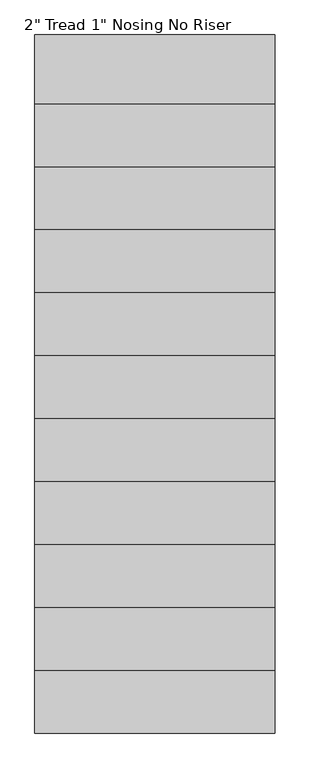
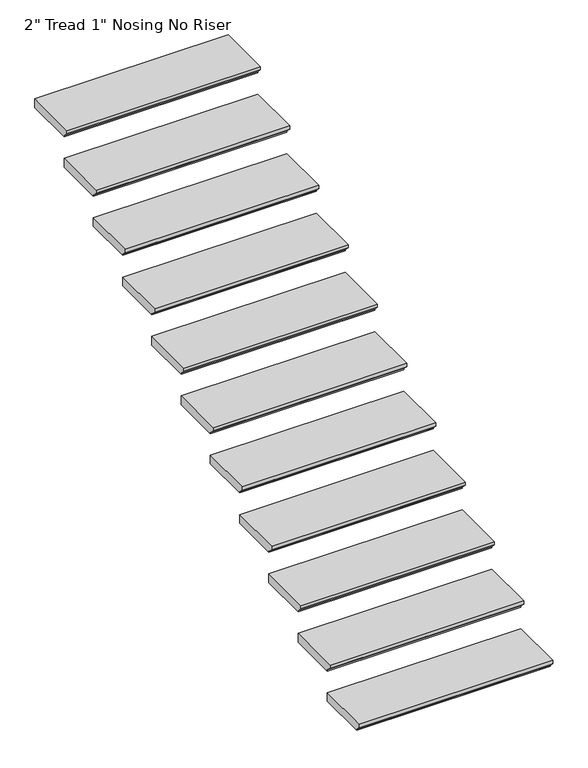
"""IFC4 building model written with IfcOpenShell, lengths in millimetres: stair flight geometry."""

import ifcopenshell
import ifcopenshell.guid

model = None  # the IFC model being written
_history = None  # IfcOwnerHistory: only IFC2X3 demands one
_inside = {}  # id of a spatial element -> (the spatial element, [elements in it])
_under = {}  # id of a project, library or spatial element -> (it, [spatial elements below it])
_declared = {}  # id of a project -> (the project, [libraries it declares])
_typed = {}  # id of a type object -> (the type object, [elements of that type])
_made_of = {}  # id of a material, layer set ... -> (it, [elements and type objects made of it])


def new_model(schema):
    """Start an empty IFC model of exactly this schema.

    Asked for "IFC4X3", IfcOpenShell would pick the latest addendum, in which some entities
    have other attributes; the version numbers below select the first issue.
    IFC2X3 requires an IfcOwnerHistory on every rooted entity: one is made here for all.
    """
    global model, _history
    if schema == "IFC4X3":
        model = ifcopenshell.file(schema_version=(4, 3, 0, 0))
    else:
        model = ifcopenshell.file(schema=schema)
    _inside.clear()
    _under.clear()
    _declared.clear()
    _typed.clear()
    _made_of.clear()
    _history = None
    if model.schema == "IFC2X3":
        org = make("IfcOrganization", Name="unknown")
        user = make(
            "IfcPersonAndOrganization",
            ThePerson=make("IfcPerson", FamilyName="unknown"),
            TheOrganization=org,
        )
        app = make(
            "IfcApplication",
            ApplicationDeveloper=org,
            Version="unknown",
            ApplicationFullName="unknown",
            ApplicationIdentifier="unknown",
        )
        _history = make(
            "IfcOwnerHistory",
            OwningUser=user,
            OwningApplication=app,
            ChangeAction="ADDED",
            CreationDate=0,
        )
    return model


def make(cls, **values):
    """One entity of the class cls with the attributes given. An attribute that is None is left unset."""
    return model.create_entity(
        cls, **{name: value for name, value in values.items() if value is not None}
    )


def rooted(cls, **values):
    """An entity with a GlobalId (a new one), such as an element, a storey or a relation."""
    return make(cls, GlobalId=ifcopenshell.guid.new(), OwnerHistory=_history, **values)


def si_unit(unit_type, name, prefix=None):
    """IfcSIUnit, for example si_unit("LENGTHUNIT", "METRE", prefix="MILLI")."""
    return make("IfcSIUnit", UnitType=unit_type, Prefix=prefix, Name=name)


def assignment(units):
    """IfcUnitAssignment: the units of a project."""
    return None if units is None else make("IfcUnitAssignment", Units=units)


def point(xyz):
    """IfcCartesianPoint."""
    return None if xyz is None else make("IfcCartesianPoint", Coordinates=xyz)


def direction(xyz):
    """IfcDirection."""
    return None if xyz is None else make("IfcDirection", DirectionRatios=xyz)


def frame(location, z_axis=None, x_axis=None):
    """IfcAxis2Placement3D, a coordinate frame: its origin and axes. An axis left out is left unset."""
    return make(
        "IfcAxis2Placement3D",
        Location=point(location),
        Axis=direction(z_axis),
        RefDirection=direction(x_axis),
    )


def origin():
    """The frame at (0, 0, 0) with its axes left unset."""
    return frame((0.0, 0.0, 0.0))


def place(relative_to, where):
    """IfcLocalPlacement: puts the frame where relative to a parent placement (None: the world)."""
    return make(
        "IfcLocalPlacement", PlacementRelTo=relative_to, RelativePlacement=where
    )


def context(
    kind, dimensions, precision=None, world=None, true_north=None, identifier=None
):
    """IfcGeometricRepresentationContext, for example the 3D "Model" context."""
    return make(
        "IfcGeometricRepresentationContext",
        ContextIdentifier=identifier,
        ContextType=kind,
        CoordinateSpaceDimension=dimensions,
        Precision=precision,
        WorldCoordinateSystem=world,
        TrueNorth=true_north,
    )


def project(units=None, contexts=None):
    """IfcProject with its units and contexts."""
    return rooted(
        "IfcProject",
        Name="project",
        RepresentationContexts=contexts,
        UnitsInContext=assignment(units),
    )


def spatial(cls, under=None, at=None, **own):
    """A site, building, storey or space (cls), placed at a placement, below another one or the project."""
    s = rooted(cls, ObjectPlacement=at, **own)
    if under is not None:
        _under.setdefault(under.id(), (under, []))[1].append(s)
    return s


def faces_of(points, faces, orient=None, outer=None):
    """IfcFace entities. A face is a list of loops; a loop is a list of indices into points, from 0.

    orient and outer hold one flag for each loop. By default every Orientation is true, the
    first loop of a face is its IfcFaceOuterBound and the others are IfcFaceBound.
    """
    made = []
    for i, loops in enumerate(faces):
        bounds = []
        for j, loop in enumerate(loops):
            is_outer = j == 0 if outer is None else outer[i][j]
            bounds.append(
                make(
                    "IfcFaceOuterBound" if is_outer else "IfcFaceBound",
                    Bound=make("IfcPolyLoop", Polygon=[points[k] for k in loop]),
                    Orientation=True if orient is None else orient[i][j],
                )
            )
        made.append(make("IfcFace", Bounds=bounds))
    return made


def faceted_brep(points, faces, orient=None, outer=None, voids=None):
    """IfcFacetedBrep: a solid bounded by flat faces; with voids (closed shells), ...WithVoids."""
    shared = [point(p) for p in points]
    hull = make("IfcClosedShell", CfsFaces=faces_of(shared, faces, orient, outer))
    if voids is None:
        return make("IfcFacetedBrep", Outer=hull)
    return make(
        "IfcFacetedBrepWithVoids",
        Outer=hull,
        Voids=[
            make(cls, CfsFaces=faces_of(shared, fs, o, b)) for cls, fs, o, b in voids
        ],
    )


def shape(context_of_items, identifier, shape_type, items):
    """IfcShapeRepresentation: the items that make up one representation, for example the "Body"."""
    return make(
        "IfcShapeRepresentation",
        ContextOfItems=context_of_items,
        RepresentationIdentifier=identifier,
        RepresentationType=shape_type,
        Items=items,
    )


def source(mapping_origin, context_of_items, identifier, shape_type, items):
    """IfcRepresentationMap: a shape defined once, which mapped items show again and again."""
    return make(
        "IfcRepresentationMap",
        MappingOrigin=mapping_origin,
        MappedRepresentation=shape(context_of_items, identifier, shape_type, items),
    )


def transform(
    local_origin,
    x_axis=None,
    y_axis=None,
    z_axis=None,
    scale=None,
    scale2=None,
    scale3=None,
    uniform=True,
):
    """IfcCartesianTransformationOperator3D, or its non-uniform kind. x_axis, y_axis, z_axis: its Axis1, 2, 3."""
    if uniform:
        return make(
            "IfcCartesianTransformationOperator3D",
            Axis1=direction(x_axis),
            Axis2=direction(y_axis),
            LocalOrigin=point(local_origin),
            Scale=scale,
            Axis3=direction(z_axis),
        )
    return make(
        "IfcCartesianTransformationOperator3DnonUniform",
        Axis1=direction(x_axis),
        Axis2=direction(y_axis),
        LocalOrigin=point(local_origin),
        Scale=scale,
        Axis3=direction(z_axis),
        Scale2=scale2,
        Scale3=scale3,
    )


def mapped(mapping_source, mapping_target):
    """IfcMappedItem: shows the shape of a source again, moved by a transform."""
    return make(
        "IfcMappedItem", MappingSource=mapping_source, MappingTarget=mapping_target
    )


def made_of(thing, what):
    """Note that an element or type object is made of a material, layer set ...; save() writes the relation."""
    if what is not None:
        _made_of.setdefault(what.id(), (what, []))[1].append(thing)
    return thing


def element(
    cls,
    number,
    at=None,
    inside=None,
    cuts=None,
    type_object=None,
    material=None,
    context=None,
    identifier="Body",
    shape_type=None,
    held_by="IfcProductDefinitionShape",
    body=None,
    shapes=None,
    **own,
):
    """One element of the class cls, such as IfcWall. Its Tag is "e" and its number.

    at: its placement. inside: the storey or other place that contains it. cuts: it is an
    opening in that element (IfcRelVoidsElement). A single representation is given by context,
    identifier, shape_type and body (its items); several are given by shapes. held_by: the class
    of the entity that holds the representations. save() writes the other relations.
    """
    e = rooted(cls, Tag="e%d" % number, ObjectPlacement=at, **own)
    if body is not None:
        shapes = [shape(context, identifier, shape_type, body)]
    if shapes is not None:
        e.Representation = make(held_by, Representations=shapes)
    if inside is not None:
        _inside.setdefault(inside.id(), (inside, []))[1].append(e)
    if cuts is not None:
        rooted(
            "IfcRelVoidsElement", RelatingBuildingElement=cuts, RelatedOpeningElement=e
        )
    if type_object is not None:
        _typed.setdefault(type_object.id(), (type_object, []))[1].append(e)
    return made_of(e, material)


def aggregate(whole, parts):
    """IfcRelAggregates: a whole, such as a stair, and the parts it consists of."""
    return rooted("IfcRelAggregates", RelatingObject=whole, RelatedObjects=parts)


def save(model, path):
    """Write the relations noted so far, then the file.

    IfcRelAggregates (storeys below a building ...), IfcRelContainedInSpatialStructure (elements
    in a storey), IfcRelDefinesByType, IfcRelAssociatesMaterial and IfcRelDeclares: one each for
    every whole, place, type object, material and project.
    """
    for whole, parts in _under.values():
        aggregate(whole, parts)
    for where, things in _inside.values():
        rooted(
            "IfcRelContainedInSpatialStructure",
            RelatedElements=things,
            RelatingStructure=where,
        )
    for kind, things in _typed.values():
        rooted("IfcRelDefinesByType", RelatedObjects=things, RelatingType=kind)
    for what, things in _made_of.values():
        rooted("IfcRelAssociatesMaterial", RelatedObjects=things, RelatingMaterial=what)
    for by, libraries in _declared.values():
        rooted("IfcRelDeclares", RelatingContext=by, RelatedDefinitions=libraries)
    model.write(path)


def stair_flight_8578e766(model_context):
    return source(origin(), model_context, "Body", "Brep", [
        faceted_brep([(-7676.1954607, -1875.4304995, 30637.6456522), (-7676.1954607, -1875.4304995, 30656.6956522), (-8742.9954607, -1875.4304995, 30656.6956522), (-8742.9954607, -1875.4304995, 30637.6456522), (-7676.1954607, -1850.0304995, 30612.2456522), (-8742.9954607, -1850.0304995, 30612.2456522), (-7676.1954607, -1570.6304995, 30656.6956522), (-8742.9954607, -1570.6304995, 30656.6956522), (-8742.9954607, -1850.0304995, 30605.8956522), (-8742.9954607, -1570.6304995, 30605.8956522), (-7676.1954607, -1570.6304995, 30605.8956522), (-7676.1954607, -1850.0304995, 30605.8956522)], [[[0, 1, 2, 3]], [[4, 0, 3, 5]], [[2, 1, 6, 7]], [[8, 9, 10, 11]], [[2, 7, 9, 8, 5, 3]], [[8, 11, 4, 5]], [[6, 1, 0, 4, 11, 10]], [[7, 6, 10, 9]]]),
        faceted_brep([(-8742.9954607, -1596.0304995, 30833.3913043), (-7676.1954607, -1596.0304995, 30833.3913043), (-7676.1954607, -1291.2304995, 30833.3913043), (-8742.9954607, -1291.2304995, 30833.3913043), (-8742.9954607, -1570.6304995, 30782.5913043), (-8742.9954607, -1291.2304995, 30782.5913043), (-7676.1954607, -1291.2304995, 30782.5913043), (-7676.1954607, -1570.6304995, 30782.5913043), (-8742.9954607, -1570.6304995, 30788.9413043), (-8742.9954607, -1596.0304995, 30814.3413043), (-7676.1954607, -1570.6304995, 30788.9413043), (-7676.1954607, -1596.0304995, 30814.3413043)], [[[0, 1, 2, 3]], [[4, 5, 6, 7]], [[0, 3, 5, 4, 8, 9]], [[4, 7, 10, 8]], [[2, 1, 11, 10, 7, 6]], [[3, 2, 6, 5]], [[11, 1, 0, 9]], [[10, 11, 9, 8]]]),
        faceted_brep([(-8742.9954607, -1316.6304995, 31010.0869565), (-7676.1954607, -1316.6304995, 31010.0869565), (-7676.1954607, -1011.8304995, 31010.0869565), (-8742.9954607, -1011.8304995, 31010.0869565), (-8742.9954607, -1291.2304995, 30959.2869565), (-8742.9954607, -1011.8304995, 30959.2869565), (-7676.1954607, -1011.8304995, 30959.2869565), (-7676.1954607, -1291.2304995, 30959.2869565), (-8742.9954607, -1291.2304995, 30965.6369565), (-8742.9954607, -1316.6304995, 30991.0369565), (-7676.1954607, -1291.2304995, 30965.6369565), (-7676.1954607, -1316.6304995, 30991.0369565)], [[[0, 1, 2, 3]], [[4, 5, 6, 7]], [[0, 3, 5, 4, 8, 9]], [[4, 7, 10, 8]], [[2, 1, 11, 10, 7, 6]], [[3, 2, 6, 5]], [[11, 1, 0, 9]], [[10, 11, 9, 8]]]),
        faceted_brep([(-8742.9954607, -1037.2304995, 31186.7826087), (-7676.1954607, -1037.2304995, 31186.7826087), (-7676.1954607, -732.4304995, 31186.7826087), (-8742.9954607, -732.4304995, 31186.7826087), (-8742.9954607, -1011.8304995, 31135.9826087), (-8742.9954607, -732.4304995, 31135.9826087), (-7676.1954607, -732.4304995, 31135.9826087), (-7676.1954607, -1011.8304995, 31135.9826087), (-8742.9954607, -1011.8304995, 31142.3326087), (-8742.9954607, -1037.2304995, 31167.7326087), (-7676.1954607, -1011.8304995, 31142.3326087), (-7676.1954607, -1037.2304995, 31167.7326087)], [[[0, 1, 2, 3]], [[4, 5, 6, 7]], [[0, 3, 5, 4, 8, 9]], [[4, 7, 10, 8]], [[2, 1, 11, 10, 7, 6]], [[3, 2, 6, 5]], [[11, 1, 0, 9]], [[10, 11, 9, 8]]]),
        faceted_brep([(-8742.9954607, -757.8304995, 31363.4782609), (-7676.1954607, -757.8304995, 31363.4782609), (-7676.1954607, -453.0304995, 31363.4782609), (-8742.9954607, -453.0304995, 31363.4782609), (-8742.9954607, -732.4304995, 31312.6782609), (-8742.9954607, -453.0304995, 31312.6782609), (-7676.1954607, -453.0304995, 31312.6782609), (-7676.1954607, -732.4304995, 31312.6782609), (-8742.9954607, -732.4304995, 31319.0282609), (-8742.9954607, -757.8304995, 31344.4282609), (-7676.1954607, -732.4304995, 31319.0282609), (-7676.1954607, -757.8304995, 31344.4282609)], [[[0, 1, 2, 3]], [[4, 5, 6, 7]], [[0, 3, 5, 4, 8, 9]], [[4, 7, 10, 8]], [[2, 1, 11, 10, 7, 6]], [[3, 2, 6, 5]], [[11, 1, 0, 9]], [[10, 11, 9, 8]]]),
        faceted_brep([(-8742.9954607, -478.4304995, 31540.173913), (-7676.1954607, -478.4304995, 31540.173913), (-7676.1954607, -173.6304995, 31540.173913), (-8742.9954607, -173.6304995, 31540.173913), (-8742.9954607, -453.0304995, 31489.373913), (-8742.9954607, -173.6304995, 31489.373913), (-7676.1954607, -173.6304995, 31489.373913), (-7676.1954607, -453.0304995, 31489.373913), (-8742.9954607, -453.0304995, 31495.723913), (-8742.9954607, -478.4304995, 31521.123913), (-7676.1954607, -453.0304995, 31495.723913), (-7676.1954607, -478.4304995, 31521.123913)], [[[0, 1, 2, 3]], [[4, 5, 6, 7]], [[0, 3, 5, 4, 8, 9]], [[4, 7, 10, 8]], [[2, 1, 11, 10, 7, 6]], [[3, 2, 6, 5]], [[11, 1, 0, 9]], [[10, 11, 9, 8]]]),
        faceted_brep([(-8742.9954607, -199.0304995, 31716.8695652), (-7676.1954607, -199.0304995, 31716.8695652), (-7676.1954607, 105.7695005, 31716.8695652), (-8742.9954607, 105.7695005, 31716.8695652), (-8742.9954607, -173.6304995, 31666.0695652), (-8742.9954607, 105.7695005, 31666.0695652), (-7676.1954607, 105.7695005, 31666.0695652), (-7676.1954607, -173.6304995, 31666.0695652), (-8742.9954607, -173.6304995, 31672.4195652), (-8742.9954607, -199.0304995, 31697.8195652), (-7676.1954607, -173.6304995, 31672.4195652), (-7676.1954607, -199.0304995, 31697.8195652)], [[[0, 1, 2, 3]], [[4, 5, 6, 7]], [[0, 3, 5, 4, 8, 9]], [[4, 7, 10, 8]], [[2, 1, 11, 10, 7, 6]], [[3, 2, 6, 5]], [[11, 1, 0, 9]], [[10, 11, 9, 8]]]),
        faceted_brep([(-8742.9954607, 80.3695005, 31893.5652174), (-7676.1954607, 80.3695005, 31893.5652174), (-7676.1954607, 385.1695005, 31893.5652174), (-8742.9954607, 385.1695005, 31893.5652174), (-8742.9954607, 105.7695005, 31842.7652174), (-8742.9954607, 385.1695005, 31842.7652174), (-7676.1954607, 385.1695005, 31842.7652174), (-7676.1954607, 105.7695005, 31842.7652174), (-8742.9954607, 105.7695005, 31849.1152174), (-8742.9954607, 80.3695005, 31874.5152174), (-7676.1954607, 105.7695005, 31849.1152174), (-7676.1954607, 80.3695005, 31874.5152174)], [[[0, 1, 2, 3]], [[4, 5, 6, 7]], [[0, 3, 5, 4, 8, 9]], [[4, 7, 10, 8]], [[2, 1, 11, 10, 7, 6]], [[3, 2, 6, 5]], [[11, 1, 0, 9]], [[10, 11, 9, 8]]]),
        faceted_brep([(-8742.9954607, 359.7695005, 32070.2608696), (-7676.1954607, 359.7695005, 32070.2608696), (-7676.1954607, 664.5695005, 32070.2608696), (-8742.9954607, 664.5695005, 32070.2608696), (-8742.9954607, 385.1695005, 32019.4608696), (-8742.9954607, 664.5695005, 32019.4608696), (-7676.1954607, 664.5695005, 32019.4608696), (-7676.1954607, 385.1695005, 32019.4608696), (-8742.9954607, 385.1695005, 32025.8108696), (-8742.9954607, 359.7695005, 32051.2108696), (-7676.1954607, 385.1695005, 32025.8108696), (-7676.1954607, 359.7695005, 32051.2108696)], [[[0, 1, 2, 3]], [[4, 5, 6, 7]], [[0, 3, 5, 4, 8, 9]], [[4, 7, 10, 8]], [[2, 1, 11, 10, 7, 6]], [[3, 2, 6, 5]], [[11, 1, 0, 9]], [[10, 11, 9, 8]]]),
        faceted_brep([(-8742.9954607, 639.1695005, 32246.9565217), (-7676.1954607, 639.1695005, 32246.9565217), (-7676.1954607, 943.9695005, 32246.9565217), (-8742.9954607, 943.9695005, 32246.9565217), (-8742.9954607, 664.5695005, 32196.1565217), (-8742.9954607, 943.9695005, 32196.1565217), (-7676.1954607, 943.9695005, 32196.1565217), (-7676.1954607, 664.5695005, 32196.1565217), (-8742.9954607, 664.5695005, 32202.5065217), (-8742.9954607, 639.1695005, 32227.9065217), (-7676.1954607, 664.5695005, 32202.5065217), (-7676.1954607, 639.1695005, 32227.9065217)], [[[0, 1, 2, 3]], [[4, 5, 6, 7]], [[0, 3, 5, 4, 8, 9]], [[4, 7, 10, 8]], [[2, 1, 11, 10, 7, 6]], [[3, 2, 6, 5]], [[11, 1, 0, 9]], [[10, 11, 9, 8]]]),
        faceted_brep([(-8742.9954607, 918.5695005, 32423.6521739), (-7676.1954607, 918.5695005, 32423.6521739), (-7676.1954607, 1197.9695005, 32423.6521739), (-7676.1954607, 1223.3695005, 32423.6521739), (-8742.9954607, 1223.3695005, 32423.6521739), (-8742.9954607, 943.9695005, 32372.8521739), (-8742.9954607, 1223.3695005, 32372.8521739), (-7676.1954607, 1223.3695005, 32372.8521739), (-7676.1954607, 1197.9695005, 32372.8521739), (-7676.1954607, 943.9695005, 32372.8521739), (-8742.9954607, 943.9695005, 32379.2021739), (-8742.9954607, 918.5695005, 32404.6021739), (-7676.1954607, 943.9695005, 32379.2021739), (-7676.1954607, 918.5695005, 32404.6021739)], [[[0, 1, 2, 3, 4]], [[5, 6, 7, 8, 9]], [[0, 4, 6, 5, 10, 11]], [[5, 9, 12, 10]], [[2, 1, 13, 12, 9, 8]], [[3, 2, 8, 7]], [[4, 3, 7, 6]], [[13, 1, 0, 11]], [[12, 13, 11, 10]]]),
    ])


if __name__ == "__main__":
    model = new_model("IFC4")
    model_context = context("Model", 3, world=origin())
    ifc_project = project(units=[si_unit("LENGTHUNIT", "METRE", prefix="MILLI")], contexts=[model_context])
    site = spatial("IfcSite", under=ifc_project)
    building = spatial("IfcBuilding", under=site)
    placement = place(None, origin())
    stair_flight_shape = stair_flight_8578e766(model_context)
    element("IfcStairFlight", 1, ObjectType="2\" Tread 1\" Nosing No Riser", at=placement, inside=building, context=model_context, shape_type="MappedRepresentation", body=[
        mapped(stair_flight_shape, transform((0.0, 0.0, 0.0), x_axis=(1.0, 0.0, 0.0), y_axis=(0.0, 1.0, 0.0), z_axis=(0.0, 0.0, 1.0))),
    ])
    save(model, "model.ifc")
